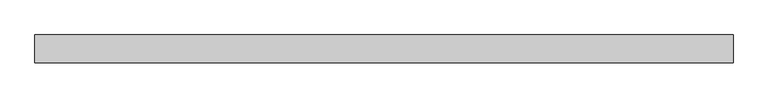
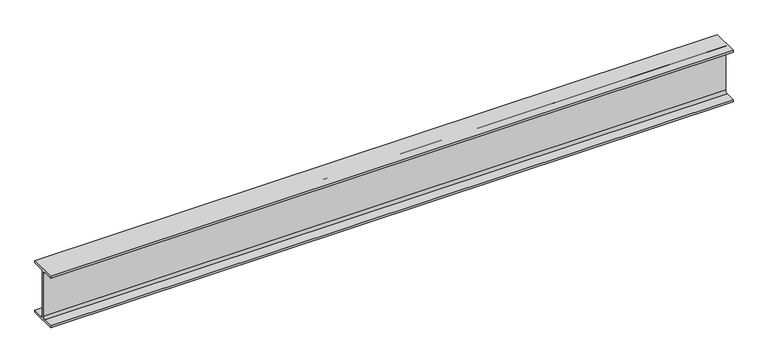
"""IFC4 building model written with IfcOpenShell, lengths in millimetres: beam geometry, 0912_Steel Framing_H-KSD3502 : H_SB_ASB_H-250x125x6x9."""

from ifc_helpers import new_model, si_unit, point, frame, frame_2d, origin, place, context, project, spatial, polyline, circle_curve, trimmed, segment, composite_curve, outline, extrude, source, transform, mapped, element, save


def beam_894be9a4(model_context):
    return source(origin(), model_context, "Body", "SweptSolid", [
        extrude(outline(composite_curve([segment(polyline([(62.5, -116.0), (62.5, -125.0), (-62.5, -125.0), (-62.5, -116.0), (-15.0, -116.0)]), True, "CONTINUOUS"), segment(trimmed(circle_curve(frame_2d((-15.0, -104.0)), 12.0), [point((-15.0, -116.0))], [point((-3.0, -104.0))], True, "CARTESIAN"), True, "CONTINUOUS"), segment(polyline([(-3.0, -104.0), (-3.0, 104.0)]), True, "CONTINUOUS"), segment(trimmed(circle_curve(frame_2d((-15.0, 104.0)), 12.0), [point((-3.0, 104.0))], [point((-15.0, 116.0))], True, "CARTESIAN"), True, "CONTINUOUS"), segment(polyline([(-15.0, 116.0), (-62.5, 116.0), (-62.5, 125.0), (62.5, 125.0), (62.5, 116.0), (15.0, 116.0)]), True, "CONTINUOUS"), segment(trimmed(circle_curve(frame_2d((15.0, 104.0)), 12.0), [point((15.0, 116.0))], [point((3.0, 104.0))], True, "CARTESIAN"), True, "CONTINUOUS"), segment(polyline([(3.0, 104.0), (3.0, -104.0)]), True, "CONTINUOUS"), segment(trimmed(circle_curve(frame_2d((15.0, -104.0)), 12.0), [point((3.0, -104.0))], [point((15.0, -116.0))], True, "CARTESIAN"), True, "CONTINUOUS"), segment(polyline([(15.0, -116.0), (62.5, -116.0)]), True, "CONTINUOUS")], self_intersect=False)), frame((-1494.4958478, 0.0, 0.0), z_axis=(1.0, 0.0, 0.0), x_axis=(0.0, 1.0, 0.0)), (0.0, 0.0, 1.0), 3149.2958913),
    ])


if __name__ == "__main__":
    model = new_model("IFC4")
    model_context = context("Model", 3, world=origin())
    ifc_project = project(units=[si_unit("LENGTHUNIT", "METRE", prefix="MILLI")], contexts=[model_context])
    site = spatial("IfcSite", under=ifc_project)
    building = spatial("IfcBuilding", under=site)
    placement = place(None, origin())
    beam_shape = beam_894be9a4(model_context)
    element("IfcBeam", 1, ObjectType="0912_Steel Framing_H-KSD3502 : H_SB_ASB_H-250x125x6x9", at=placement, inside=building, context=model_context, shape_type="MappedRepresentation", body=[
        mapped(beam_shape, transform((0.0, 0.0, 0.0), x_axis=(1.0, 0.0, 0.0), y_axis=(0.0, 1.0, 0.0), z_axis=(0.0, 0.0, 1.0))),
    ])
    save(model, "model.ifc")

# Revit data of these elements
# Type "0912_Steel Framing_H-KSD3502 : H_SB_ASB_H-250x125x6x9"
#   H_WM Code_1 = "S01AA003-00001 | Main Steel Structure Fabrication Work | Shelter/Building | Light Steel - Standard (30KG/M>Weight) | Material: (   )"
#   H_WM Code_2 = "S03AA029-00001 | Main Steel Structure Erection Work | Shelter/Building | Light Steel (30KG/M>Weight) | Material: (   )"
#   H_WM Code_3 = "S01AA010-00001 | Main Steel Structure Fabrication Work | Shelter/Building | Steel Painting/Coating | for Non-Fireproofed Steel Surface, Surface Preparation, Primer, Second & Final Coat | Material: (   )"
#   H_Q'ty Cal Type Tag = "SB-Q2"
#   Width = 12.5 cm
#   Web Thickness = 0.6 cm
#   Web Fillet = 1.2 cm
#   Warping Constant = 42539.8 cm⁶
#   W = 0
#   Torsional Moment of Inertia = 7.8102 cm⁴
#   Section Area = 37.66 cm²
#   Plastic Modulus weak axis = 73.1 cm³
#   Plastic Modulus strong axis = 366.0 cm³
#   Perimeter = 0.97 m²/m
#   Nominal Weight = 29.60 kgf/m
#   Moment of Inertia weak axis = 294.00 cm⁴
#   Moment of Inertia strong axis = 4050.00 cm⁴
#   Height = 25.0 cm
#   Flange Thickness = 0.9 cm
#   Elastic Modulus weak axis = 47.0 cm³
#   Elastic Modulus strong axis = 324.0 cm³
#   Centroid Vertical = 12.5 cm
#   Centroid Horizontal = 6.25 cm
#   Ix = 40500000
#   Length [instance default] = 1.5240 m
#   Zx = 366000
#   b = 0.1250 m
#   h = 0.2500 m
#   r = 0.0120 m
#   s = 0.0060 m
#   t = 0.0090 m
#   A = 0.003766 m²
#   Structural Material [instance default] = Steel, 45-345
#   Assembly Code = ""
# Element 1 (IfcBeam, "0912_Steel Framing_H-KSD3502 : H_SB_ASB_H-250x125x6x9")
#   Structural Material = none
# Materials
#   "Steel, 45-345": class "Metal", colour RGB 189 187 185, transparency 0, Description = "Steel 345 MPa", Cost = 0
